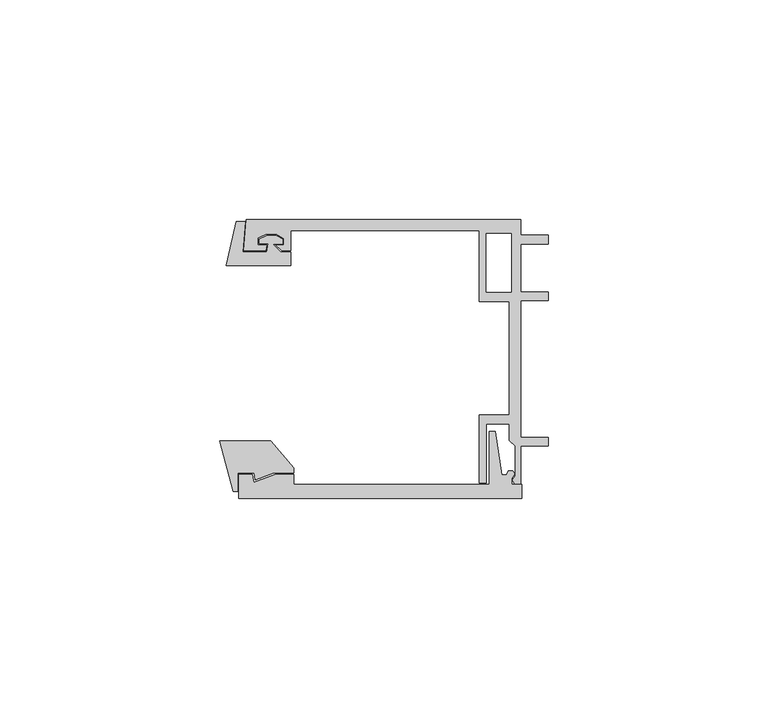
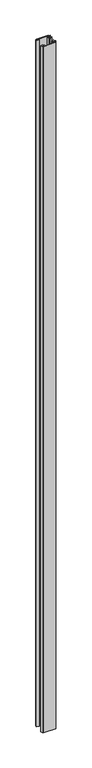
"""IFC4 building model written with IfcOpenShell, lengths in millimetres: proxy geometry, Generic Models 2:Generic Models 2:310765:Generic Models 2:310765 : Generic Models 2:Generic Models 2:310765:6 : Generic Models 2:Generic Models 2:310765:Generic Models 2:310765 : Generic Models 2:Generic Models 2:310765:300385."""

from ifc_helpers import new_model, si_unit, frame, origin, place, context, project, spatial, polyline, outline, extrude, source, transform, mapped, element, save


def generic_models_96f1aa04(model_context):
    return source(origin(), model_context, "Body", "SweptSolid", [
        extrude(outline(polyline([(592746.3712702, -579078.5739799), (592747.3211391, -579078.5247354), (592747.8148424, -579079.2652904), (592747.15618, -579080.2786171), (592747.15618, -579081.6864938), (592749.468505, -579081.6864938), (592749.468505, -579084.8288841), (592684.9605685, -579084.8288841), (592684.9605685, -579079.3741689), (592688.1029588, -579079.3741689), (592688.3994107, -579081.1528804), (592693.2612221, -579079.3741689), (592697.5301296, -579079.3741689), (592697.5301296, -579081.6864938), (592742.0572071, -579081.6864938), (592742.0572071, -579069.5319653), (592743.429356, -579069.5319653), (592744.8438551, -579079.4334593), (592745.8946421, -579079.4334593), (592746.3712702, -579078.5739799)])), frame((0.0, 0.0, 29.36875), z_axis=(0.0, 0.0, 1.0), x_axis=(1.0, 0.0, 0.0)), (0.0, 0.0, 1.0), 3670.2203961),
        extrude(outline(polyline([(592683.7242356, -579083.2164454), (592680.6758501, -579071.7849999), (592692.2814632, -579071.7849999), (592697.5301296, -579077.8782793), (592697.5301296, -579079.0835833), (592693.0009934, -579079.0835833), (592688.7860927, -579080.6256201), (592688.5290865, -579079.0835833), (592684.7628487, -579079.0835833), (592684.7628487, -579083.2164454), (592683.7242356, -579083.2164454)])), frame((0.0, 0.0, 29.36875), z_axis=(0.0, 0.0, 1.0), x_axis=(1.0, 0.0, 0.0)), (0.0, 0.0, 1.0), 3670.2203961),
        extrude(outline(polyline([(592696.818645, -579023.8783705), (592696.818645, -579028.44373), (592694.7730504, -579028.44373), (592693.4687779, -579027.1393416), (592695.2770951, -579027.1393416), (592695.2770951, -579025.657082), (592693.5557477, -579024.6632617), (592691.2743287, -579024.6632617), (592689.3755356, -579025.5486834), (592689.3755356, -579027.1393416), (592691.4087591, -579027.1393416), (592691.1860587, -579028.44373), (592686.1463761, -579028.44373), (592686.7448211, -579021.3288841), (592749.1720531, -579021.3288841), (592749.1720531, -579024.8863071), (592755.4568336, -579024.8863071), (592755.4568336, -579026.9021801), (592749.1720531, -579026.9021801), (592749.1720531, -579037.8116105), (592755.4568336, -579037.8116105), (592755.4568336, -579039.8274835), (592749.1720531, -579039.8274835), (592749.1720531, -579070.8956441), (592755.4568336, -579070.8956441), (592755.4568336, -579072.9115171), (592749.1720531, -579072.9115171), (592749.1720531, -579081.5086227), (592747.8083743, -579081.5086227), (592747.2747608, -579080.6785573), (592747.926955, -579079.7299112), (592747.926955, -579072.9115171), (592746.6225666, -579071.6071287), (592746.6225666, -579067.8718346), (592741.2864321, -579067.8718346), (592741.2864321, -579081.3307515), (592739.7448822, -579081.3307515), (592739.7448822, -579065.8559616), (592746.6225666, -579065.8559616), (592746.6225666, -579039.9460643), (592739.7448822, -579039.9460643), (592739.7448822, -579023.8783705), (592696.818645, -579023.8783705)]), holes=[polyline([(592747.0375993, -579024.4712744), (592741.2864321, -579024.4712744), (592741.2864321, -579037.8116105), (592747.0375993, -579037.8116105), (592747.0375993, -579024.4712744)])]), frame((0.0, 0.0, 29.36875), z_axis=(0.0, 0.0, 1.0), x_axis=(1.0, 0.0, 0.0)), (0.0, 0.0, 1.0), 3670.2203961),
        extrude(outline(polyline([(592682.1660262, -579031.7849999), (592684.3847904, -579021.8263604), (592686.4862053, -579021.8263604), (592685.9037947, -579028.7505755), (592691.3440945, -579028.7505755), (592691.6725229, -579026.8269234), (592689.6342596, -579026.8269234), (592689.6342596, -579025.8025744), (592691.4357431, -579024.9625289), (592693.5160416, -579024.9625289), (592695.0063819, -579025.8229772), (592695.0063819, -579026.9121641), (592692.7519937, -579026.9121641), (592694.5904051, -579028.7505755), (592696.818645, -579028.7505755), (592696.818645, -579031.7849999), (592682.1660262, -579031.7849999)])), frame((0.0, 0.0, 29.36875), z_axis=(0.0, 0.0, 1.0), x_axis=(1.0, 0.0, 0.0)), (0.0, 0.0, 1.0), 3670.2203961),
    ])


if __name__ == "__main__":
    model = new_model("IFC4")
    model_context = context("Model", 3, world=origin())
    ifc_project = project(units=[si_unit("LENGTHUNIT", "METRE", prefix="MILLI")], contexts=[model_context])
    site = spatial("IfcSite", under=ifc_project)
    building = spatial("IfcBuilding", under=site)
    placement = place(None, origin())
    generic_models_shape = generic_models_96f1aa04(model_context)
    element("IfcBuildingElementProxy", 1, Name="Generic Models 2:Generic Models 2:310765:Generic Models 2:310765 : Generic Models 2:Generic Models 2:310765:6 : Generic Models 2:Generic Models 2:310765:Generic Models 2:310765 : Generic Models 2:Generic Models 2:310765:300385", ObjectType="Generic Models 2:Generic Models 2:310765:Generic Models 2:310765 : Generic Models 2:Generic Models 2:310765:6 : Generic Models 2:Generic Models 2:310765:Generic Models 2:310765 : Generic Models 2:Generic Models 2:310765:300385", at=placement, inside=building, context=model_context, shape_type="MappedRepresentation", body=[
        mapped(generic_models_shape, transform((0.0, 0.0, 0.0), x_axis=(1.0, 0.0, 0.0), y_axis=(0.0, 1.0, 0.0), z_axis=(0.0, 0.0, 1.0))),
    ])
    save(model, "model.ifc")

# Revit data of these elements
# Type "Generic Models 2:Generic Models 2:310765:Generic Models 2:310765 : Generic Models 2:Generic Models 2:310765:6 : Generic Models 2:Generic Models 2:310765:Generic Models 2:310765 : Generic Models 2:Generic Models 2:310765:300385"
#   NameOverride = "Generic Models 2:Generic Models 2:310765:Generic Models 2:310765 : Generic Models 2:Generic Models 2:310765:300385"
#   ObjectTypeOverride = "Generic Models 2:310765 : Generic Models 2:Generic Models 2:310765"
#   Reference = "Generic Models 2"
#   Tag = "300385"
# Element 1 (IfcBuildingElementProxy, "Generic Models 2:Generic Models 2:310765:Generic Models 2:310765 : Generic Models 2:Generic Models 2:310765:6 : Generic Models 2:Generic Models 2:310765:Generic Models 2:310765 : Generic Models 2:Generic Models 2:310765:300385")
#   Materials on its faces: "THERMAL BROKEN ALUMINUM STOREFRONT FOR POLYCARBONATE"
# Materials
#   "THERMAL BROKEN ALUMINUM STOREFRONT FOR POLYCARBONATE": class "Unassigned", colour RGB 244 244 244, transparency 0, Keynote = "M07611300.01", Cost = 0
